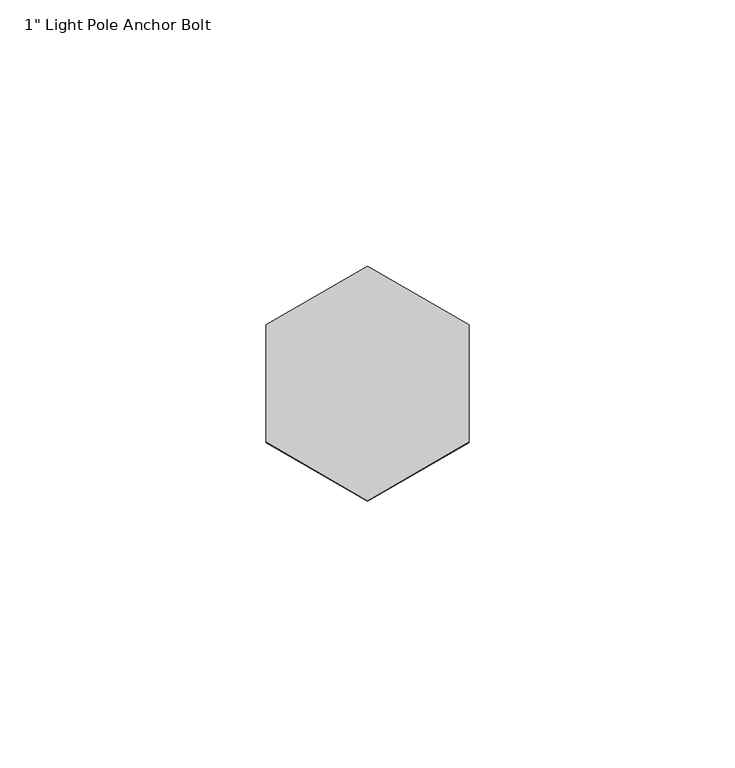
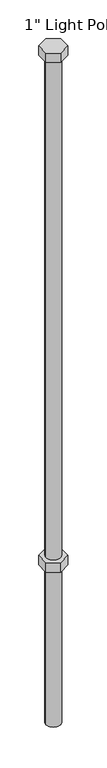
"""IFC4 building model written with IfcOpenShell, lengths in millimetres: proxy geometry."""

from ifc_helpers import new_model, si_unit, point, frame, origin, origin_with_axes, origin_2d, place, context, project, spatial, polyline, circle_curve, trimmed, segment, composite_curve, outline, extrude, source, transform, mapped, element, save


def proxy_3d40efa6(model_context):
    return source(origin(), model_context, "Body", "SweptSolid", [
        extrude(outline(polyline([(-19.05, -10.9985226), (-19.05, 10.9985226), (0.0, 21.9970453), (19.05, 10.9985226), (19.05, -10.9985226), (0.0, -21.9970453), (-19.05, -10.9985226)])), frame((0.0, 0.0, -931.465625), z_axis=(0.0, 0.0, 1.0), x_axis=(1.0, 0.0, 0.0)), (0.0, 0.0, 1.0), 17.065625),
        extrude(outline(polyline([(-19.05, 10.9985226), (0.0, 21.9970453), (19.05, 10.9985226), (19.05, -10.9985226), (0.0, -21.9970453), (-19.05, -10.9985226), (-19.05, 10.9985226)])), origin_with_axes(), (0.0, 0.0, 1.0), 17.065625),
        extrude(outline(composite_curve([segment(trimmed(circle_curve(origin_2d(), 12.7), [point((-12.7, 0.0))], [point((12.7, 0.0))], False, "CARTESIAN"), True, "CONTINUOUS"), segment(trimmed(circle_curve(origin_2d(), 12.7), [point((12.7, 0.0))], [point((-12.7, 0.0))], False, "CARTESIAN"), True, "CONTINUOUS")], self_intersect=False)), frame((0.0, 0.0, -1219.2), z_axis=(0.0, 0.0, 1.0), x_axis=(1.0, 0.0, 0.0)), (0.0, 0.0, 1.0), 1219.2),
    ])


if __name__ == "__main__":
    model = new_model("IFC4")
    model_context = context("Model", 3, world=origin())
    ifc_project = project(units=[si_unit("LENGTHUNIT", "METRE", prefix="MILLI")], contexts=[model_context])
    site = spatial("IfcSite", under=ifc_project)
    building = spatial("IfcBuilding", under=site)
    placement = place(None, origin())
    proxy_shape = proxy_3d40efa6(model_context)
    element("IfcBuildingElementProxy", 1, Name="050523 - W_P_C - Fastenings - Lag Bolt or Thru Bolt : 1\" Light Pole Anchor Bolt", ObjectType="050523 - W_P_C - Fastenings - Lag Bolt or Thru Bolt : 1\" Light Pole Anchor Bolt", at=placement, inside=building, context=model_context, shape_type="MappedRepresentation", body=[
        mapped(proxy_shape, transform((0.0, 0.0, 0.0), x_axis=(1.0, 0.0, 0.0), y_axis=(0.0, 1.0, 0.0), z_axis=(0.0, 0.0, 1.0))),
    ])
    save(model, "model.ifc")

# Revit data of these elements
# Type "050523 - W_P_C - Fastenings - Lag Bolt or Thru Bolt : 1\" Light Pole Anchor Bolt"
#   Thickness_of_Substrate [instance default] = 0' - 1"
#   Side = 0' - 0 111/128"
#   Radius = 0' - 0 1/2"
#   Length = 4' - 0"
#   Head Size = 0' - 1 1/2"
#   Head Radius = 0' - 0 3/4"
#   Head Height = 0' - 0 43/64"
#   Diameter = 0' - 1"
#   Default Elevation = 4' - 0"
#   Nut_Visibility [instance default] = yes
#   Bolt Material (Size) [instance default] = 5/8" GALV. ANCHOR BOLT @ 24" O.C. (6" MIN. EMBEDMENT)
# Element 1 (IfcBuildingElementProxy, "050523 - W_P_C - Fastenings - Lag Bolt or Thru Bolt : 1\" Light Pole Anchor Bolt")
#   Thickness_of_Substrate = 3' - 0"
#   Bolt Material (Size) = STRUCTURAL BOLTS (PAINT TO MATCH STEEL FINISH)
#   Materials on its faces: "STRUCTURAL BOLTS (PAINT TO MATCH STEEL FINISH)"
# Materials
#   "5/8\" GALV. ANCHOR BOLT @ 24\" O.C. (6\" MIN. EMBEDMENT)": class "Generic", colour RGB 120 120 120, transparency 0, Cost = 0
#   "STRUCTURAL BOLTS (PAINT TO MATCH STEEL FINISH)": class "Generic", colour RGB 120 120 120, transparency 0, Cost = 0
